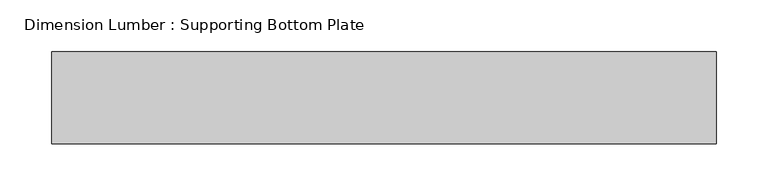
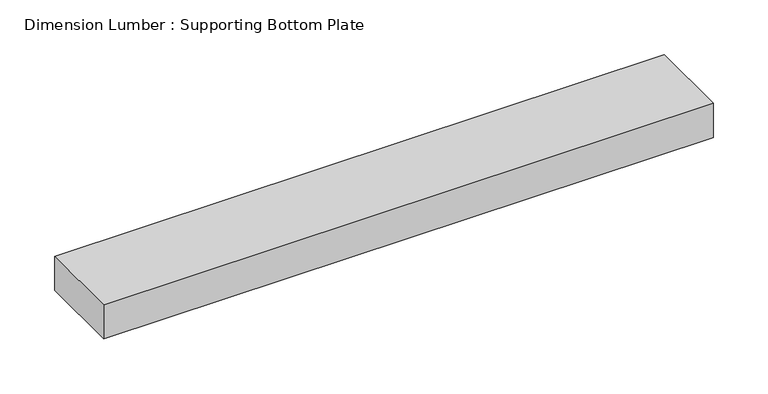
"""IFC4 building model written with IfcOpenShell, lengths in millimetres: beam geometry, Dimension Lumber : Supporting Bottom Plate."""

from ifc_helpers import new_model, si_unit, frame, origin, place, context, project, spatial, polyline, outline, extrude, source, transform, mapped, element, save


def dimension_lumber_supporting_bottom_plate_fcdf3739(model_context):
    return source(origin(), model_context, "Body", "SweptSolid", [
        extrude(outline(polyline([(352.425, 44.45), (352.425, -44.45), (-288.925, -44.45), (-288.925, 44.45), (352.425, 44.45)])), frame((0.0, 0.0, -19.05), z_axis=(0.0, 0.0, 1.0), x_axis=(1.0, 0.0, 0.0)), (0.0, 0.0, 1.0), 38.1),
    ])


if __name__ == "__main__":
    model = new_model("IFC4")
    model_context = context("Model", 3, world=origin())
    ifc_project = project(units=[si_unit("LENGTHUNIT", "METRE", prefix="MILLI")], contexts=[model_context])
    site = spatial("IfcSite", under=ifc_project)
    building = spatial("IfcBuilding", under=site)
    placement = place(None, origin())
    dimension_lumber_supporting_bottom_plate_shape = dimension_lumber_supporting_bottom_plate_fcdf3739(model_context)
    element("IfcBeam", 1, ObjectType="Dimension Lumber : Supporting Bottom Plate", at=placement, inside=building, context=model_context, shape_type="MappedRepresentation", body=[
        mapped(dimension_lumber_supporting_bottom_plate_shape, transform((0.0, 0.0, 0.0), x_axis=(1.0, 0.0, 0.0), y_axis=(0.0, 1.0, 0.0), z_axis=(0.0, 0.0, 1.0))),
    ])
    save(model, "model.ifc")

# Revit data of these elements
# Type "Dimension Lumber : Supporting Bottom Plate"
#   Assembly Code = "B10"
#   A = 0.0364583 SF
#   Length [instance default] = 5' - 0"
#   b = 0' - 3 1/2"
#   d = 0' - 1 1/2"
#   Structural Material [instance default] = Softwood, Lumber
# Element 1 (IfcBeam, "Dimension Lumber : Supporting Bottom Plate")
#   Structural Material = Douglas Fir #2
#   Materials on its faces: "Douglas Fir #2"
# Materials
#   "Softwood, Lumber": class "Wood", colour RGB 223 192 134, transparency 0, Description = "Pinus Echinata", Cost = 0
#   "Douglas Fir #2": class "Wood", colour RGB 223 192 134, transparency 0, Description = "Pinus Echinata", Cost = 0
